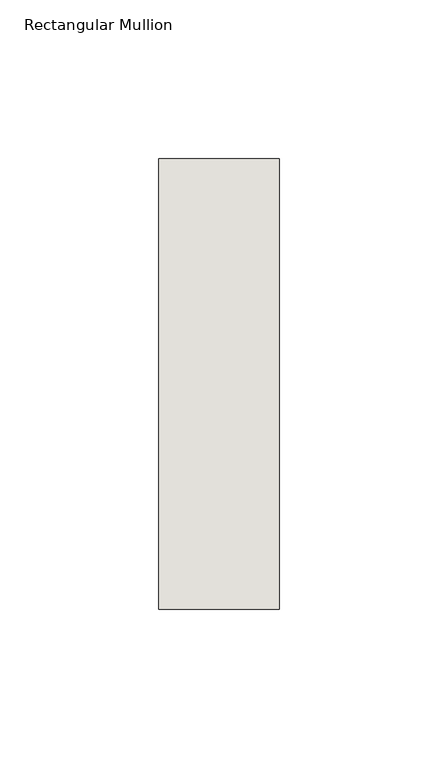
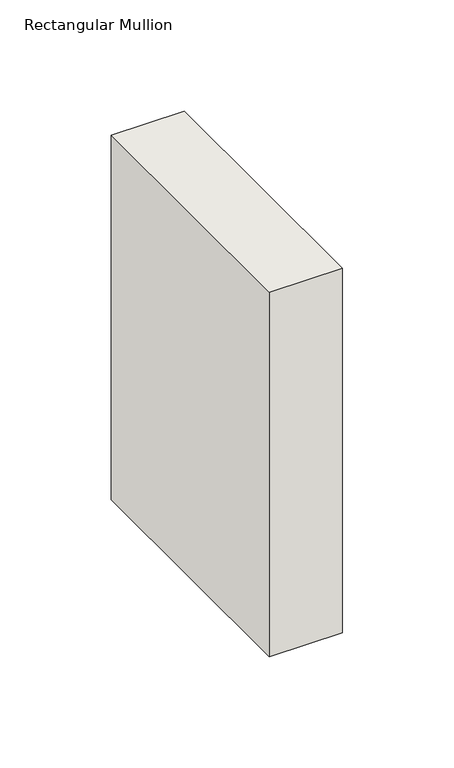
"""IFC4 building model written with IfcOpenShell, lengths in millimetres: wall geometry, Rectangular Mullion : NLRS_21_CWM_hsb-regel 38x142_gen_rsf."""

import ifcopenshell
import ifcopenshell.guid

model = None  # the IFC model being written
_history = None  # IfcOwnerHistory: only IFC2X3 demands one
_inside = {}  # id of a spatial element -> (the spatial element, [elements in it])
_under = {}  # id of a project, library or spatial element -> (it, [spatial elements below it])
_declared = {}  # id of a project -> (the project, [libraries it declares])
_typed = {}  # id of a type object -> (the type object, [elements of that type])
_made_of = {}  # id of a material, layer set ... -> (it, [elements and type objects made of it])


def new_model(schema):
    """Start an empty IFC model of exactly this schema.

    Asked for "IFC4X3", IfcOpenShell would pick the latest addendum, in which some entities
    have other attributes; the version numbers below select the first issue.
    IFC2X3 requires an IfcOwnerHistory on every rooted entity: one is made here for all.
    """
    global model, _history
    if schema == "IFC4X3":
        model = ifcopenshell.file(schema_version=(4, 3, 0, 0))
    else:
        model = ifcopenshell.file(schema=schema)
    _inside.clear()
    _under.clear()
    _declared.clear()
    _typed.clear()
    _made_of.clear()
    _history = None
    if model.schema == "IFC2X3":
        org = make("IfcOrganization", Name="unknown")
        user = make(
            "IfcPersonAndOrganization",
            ThePerson=make("IfcPerson", FamilyName="unknown"),
            TheOrganization=org,
        )
        app = make(
            "IfcApplication",
            ApplicationDeveloper=org,
            Version="unknown",
            ApplicationFullName="unknown",
            ApplicationIdentifier="unknown",
        )
        _history = make(
            "IfcOwnerHistory",
            OwningUser=user,
            OwningApplication=app,
            ChangeAction="ADDED",
            CreationDate=0,
        )
    return model


def make(cls, **values):
    """One entity of the class cls with the attributes given. An attribute that is None is left unset."""
    return model.create_entity(
        cls, **{name: value for name, value in values.items() if value is not None}
    )


def rooted(cls, **values):
    """An entity with a GlobalId (a new one), such as an element, a storey or a relation."""
    return make(cls, GlobalId=ifcopenshell.guid.new(), OwnerHistory=_history, **values)


def si_unit(unit_type, name, prefix=None):
    """IfcSIUnit, for example si_unit("LENGTHUNIT", "METRE", prefix="MILLI")."""
    return make("IfcSIUnit", UnitType=unit_type, Prefix=prefix, Name=name)


def assignment(units):
    """IfcUnitAssignment: the units of a project."""
    return None if units is None else make("IfcUnitAssignment", Units=units)


def point(xyz):
    """IfcCartesianPoint."""
    return None if xyz is None else make("IfcCartesianPoint", Coordinates=xyz)


def direction(xyz):
    """IfcDirection."""
    return None if xyz is None else make("IfcDirection", DirectionRatios=xyz)


def frame(location, z_axis=None, x_axis=None):
    """IfcAxis2Placement3D, a coordinate frame: its origin and axes. An axis left out is left unset."""
    return make(
        "IfcAxis2Placement3D",
        Location=point(location),
        Axis=direction(z_axis),
        RefDirection=direction(x_axis),
    )


def origin():
    """The frame at (0, 0, 0) with its axes left unset."""
    return frame((0.0, 0.0, 0.0))


def place(relative_to, where):
    """IfcLocalPlacement: puts the frame where relative to a parent placement (None: the world)."""
    return make(
        "IfcLocalPlacement", PlacementRelTo=relative_to, RelativePlacement=where
    )


def context(
    kind, dimensions, precision=None, world=None, true_north=None, identifier=None
):
    """IfcGeometricRepresentationContext, for example the 3D "Model" context."""
    return make(
        "IfcGeometricRepresentationContext",
        ContextIdentifier=identifier,
        ContextType=kind,
        CoordinateSpaceDimension=dimensions,
        Precision=precision,
        WorldCoordinateSystem=world,
        TrueNorth=true_north,
    )


def project(units=None, contexts=None):
    """IfcProject with its units and contexts."""
    return rooted(
        "IfcProject",
        Name="project",
        RepresentationContexts=contexts,
        UnitsInContext=assignment(units),
    )


def spatial(cls, under=None, at=None, **own):
    """A site, building, storey or space (cls), placed at a placement, below another one or the project."""
    s = rooted(cls, ObjectPlacement=at, **own)
    if under is not None:
        _under.setdefault(under.id(), (under, []))[1].append(s)
    return s


def polyline(points):
    """IfcPolyline through the points."""
    return make("IfcPolyline", Points=[point(p) for p in points])


def outline(outer, holes=None, kind="AREA"):
    """IfcArbitraryClosedProfileDef: a profile drawn as a closed curve; with holes, ...WithVoids."""
    if holes is None:
        return make("IfcArbitraryClosedProfileDef", ProfileType=kind, OuterCurve=outer)
    return make(
        "IfcArbitraryProfileDefWithVoids",
        ProfileType=kind,
        OuterCurve=outer,
        InnerCurves=holes,
    )


def extrude(swept, where, along, depth):
    """IfcExtrudedAreaSolid: the profile swept, set in the frame where, extruded along a direction by depth."""
    return make(
        "IfcExtrudedAreaSolid",
        SweptArea=swept,
        Position=where,
        ExtrudedDirection=direction(along),
        Depth=depth,
    )


def shape(context_of_items, identifier, shape_type, items):
    """IfcShapeRepresentation: the items that make up one representation, for example the "Body"."""
    return make(
        "IfcShapeRepresentation",
        ContextOfItems=context_of_items,
        RepresentationIdentifier=identifier,
        RepresentationType=shape_type,
        Items=items,
    )


def source(mapping_origin, context_of_items, identifier, shape_type, items):
    """IfcRepresentationMap: a shape defined once, which mapped items show again and again."""
    return make(
        "IfcRepresentationMap",
        MappingOrigin=mapping_origin,
        MappedRepresentation=shape(context_of_items, identifier, shape_type, items),
    )


def transform(
    local_origin,
    x_axis=None,
    y_axis=None,
    z_axis=None,
    scale=None,
    scale2=None,
    scale3=None,
    uniform=True,
):
    """IfcCartesianTransformationOperator3D, or its non-uniform kind. x_axis, y_axis, z_axis: its Axis1, 2, 3."""
    if uniform:
        return make(
            "IfcCartesianTransformationOperator3D",
            Axis1=direction(x_axis),
            Axis2=direction(y_axis),
            LocalOrigin=point(local_origin),
            Scale=scale,
            Axis3=direction(z_axis),
        )
    return make(
        "IfcCartesianTransformationOperator3DnonUniform",
        Axis1=direction(x_axis),
        Axis2=direction(y_axis),
        LocalOrigin=point(local_origin),
        Scale=scale,
        Axis3=direction(z_axis),
        Scale2=scale2,
        Scale3=scale3,
    )


def mapped(mapping_source, mapping_target):
    """IfcMappedItem: shows the shape of a source again, moved by a transform."""
    return make(
        "IfcMappedItem", MappingSource=mapping_source, MappingTarget=mapping_target
    )


def made_of(thing, what):
    """Note that an element or type object is made of a material, layer set ...; save() writes the relation."""
    if what is not None:
        _made_of.setdefault(what.id(), (what, []))[1].append(thing)
    return thing


def element(
    cls,
    number,
    at=None,
    inside=None,
    cuts=None,
    type_object=None,
    material=None,
    context=None,
    identifier="Body",
    shape_type=None,
    held_by="IfcProductDefinitionShape",
    body=None,
    shapes=None,
    **own,
):
    """One element of the class cls, such as IfcWall. Its Tag is "e" and its number.

    at: its placement. inside: the storey or other place that contains it. cuts: it is an
    opening in that element (IfcRelVoidsElement). A single representation is given by context,
    identifier, shape_type and body (its items); several are given by shapes. held_by: the class
    of the entity that holds the representations. save() writes the other relations.
    """
    e = rooted(cls, Tag="e%d" % number, ObjectPlacement=at, **own)
    if body is not None:
        shapes = [shape(context, identifier, shape_type, body)]
    if shapes is not None:
        e.Representation = make(held_by, Representations=shapes)
    if inside is not None:
        _inside.setdefault(inside.id(), (inside, []))[1].append(e)
    if cuts is not None:
        rooted(
            "IfcRelVoidsElement", RelatingBuildingElement=cuts, RelatedOpeningElement=e
        )
    if type_object is not None:
        _typed.setdefault(type_object.id(), (type_object, []))[1].append(e)
    return made_of(e, material)


def aggregate(whole, parts):
    """IfcRelAggregates: a whole, such as a stair, and the parts it consists of."""
    return rooted("IfcRelAggregates", RelatingObject=whole, RelatedObjects=parts)


def save(model, path):
    """Write the relations noted so far, then the file.

    IfcRelAggregates (storeys below a building ...), IfcRelContainedInSpatialStructure (elements
    in a storey), IfcRelDefinesByType, IfcRelAssociatesMaterial and IfcRelDeclares: one each for
    every whole, place, type object, material and project.
    """
    for whole, parts in _under.values():
        aggregate(whole, parts)
    for where, things in _inside.values():
        rooted(
            "IfcRelContainedInSpatialStructure",
            RelatedElements=things,
            RelatingStructure=where,
        )
    for kind, things in _typed.values():
        rooted("IfcRelDefinesByType", RelatedObjects=things, RelatingType=kind)
    for what, things in _made_of.values():
        rooted("IfcRelAssociatesMaterial", RelatedObjects=things, RelatingMaterial=what)
    for by, libraries in _declared.values():
        rooted("IfcRelDeclares", RelatingContext=by, RelatedDefinitions=libraries)
    model.write(path)


def rectangular_mullion_fa24708d(model_context):
    return source(origin(), model_context, "Body", "SweptSolid", [
        extrude(outline(polyline([(0.0, -71.0), (-38.0, -71.0), (-38.0, 71.0), (0.0, 71.0), (0.0, -71.0)])), frame((0.0, 0.0, -199.9999997), z_axis=(0.0, 0.0, 1.0), x_axis=(1.0, 0.0, 0.0)), (0.0, 0.0, 1.0), 199.9999997),
    ])


if __name__ == "__main__":
    model = new_model("IFC4")
    model_context = context("Model", 3, world=origin())
    ifc_project = project(units=[si_unit("LENGTHUNIT", "METRE", prefix="MILLI")], contexts=[model_context])
    site = spatial("IfcSite", under=ifc_project)
    building = spatial("IfcBuilding", under=site)
    placement = place(None, origin())
    rectangular_mullion_shape = rectangular_mullion_fa24708d(model_context)
    element("IfcWall", 1, ObjectType="Rectangular Mullion : NLRS_21_CWM_hsb-regel 38x142_gen_rsf", at=placement, inside=building, context=model_context, shape_type="MappedRepresentation", body=[
        mapped(rectangular_mullion_shape, transform((0.0, 0.0, 0.0), x_axis=(1.0, 0.0, 0.0), y_axis=(0.0, 1.0, 0.0), z_axis=(0.0, 0.0, 1.0))),
    ])
    save(model, "model.ifc")

# Revit data of these elements
# Type "Rectangular Mullion : NLRS_21_CWM_hsb-regel 38x142_gen_rsf"
#   Type IfcGUID = "07M7mRoiH1CR8m_RSKIwpF"
#   Assembly Code = "21.10"
#   IfcExportAs = "IfcWall"
#   built-in parameter 1007322 = 0.465879 (stored number, unit not read)
#   built-in parameter 1007321 = 0.062336 (stored number, unit not read)
#   built-in parameter 1007320 = 0.062336 (stored number, unit not read)
# Element 1 (IfcWall, "Rectangular Mullion : NLRS_21_CWM_hsb-regel 38x142_gen_rsf")
#   Materials on its faces: "NLRS_i2_hout naaldhout vuren_gen_rsf"
# Materials
#   "NLRS_i2_hout naaldhout vuren_gen_rsf": class "I - Hout", colour RGB 234 199 147, transparency 0, Keynote = "i2", Manufacturer = "Revit Standards Foundation", URL = "www.revitstandards.org", Description = "hout vuren", Cost = 0
